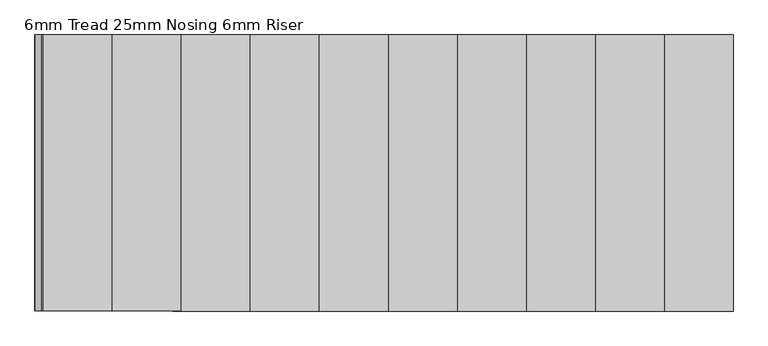
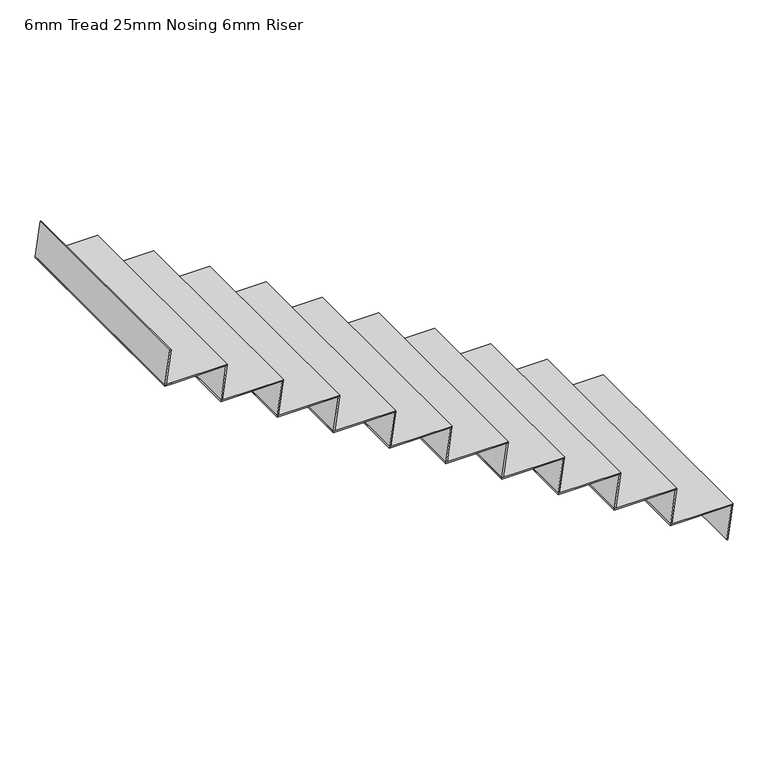
"""IFC4 building model written with IfcOpenShell, lengths in millimetres: stair flight geometry, 6mm Tread 25mm Nosing 6mm Riser."""

from ifc_helpers import new_model, si_unit, origin, place, context, project, spatial, faceted_brep, source, transform, mapped, element, save


def stair_flight_6mm_tread_25mm_nosing_6mm_riser_dd6273b0(model_context):
    return source(origin(), model_context, "Body", "Brep", [
        faceted_brep([(-13906.0599092, 11470.4345331, 8176.4705882), (-13906.9099092, 11470.4345331, 8170.4705882), (-13906.9099092, 10370.4345331, 8170.4705882), (-13906.0599092, 10370.4345331, 8176.4705882), (-13600.0, 10370.4345331, 8176.4705882), (-13600.0, 11470.4345331, 8176.4705882), (-13600.85, 11470.4345331, 8170.4705882), (-13600.85, 10370.4345331, 8170.4705882)], [[[0, 1, 2, 3]], [[3, 4, 5, 0]], [[2, 1, 6, 7]], [[4, 3, 2, 7]], [[0, 5, 6, 1]], [[5, 4, 7, 6]]]),
        faceted_brep([(-13600.85, 11470.4345331, 8170.4705882), (-13625.0, 11470.4345331, 8000.0), (-13631.0599092, 11470.4345331, 8000.0), (-13606.9099092, 11470.4345331, 8170.4705882), (-13600.85, 10370.4345331, 8170.4705882), (-13606.9099092, 10370.4345331, 8170.4705882), (-13631.0599092, 10370.4345331, 8000.0), (-13625.0, 10370.4345331, 8000.0)], [[[0, 1, 2, 3]], [[4, 5, 6, 7]], [[1, 0, 4, 7]], [[2, 1, 7, 6]], [[3, 2, 6, 5]], [[0, 3, 5, 4]]]),
        faceted_brep([(-13875.85, 11470.4345331, 8346.9411765), (-13900.0, 11470.4345331, 8176.4705882), (-13906.0599092, 11470.4345331, 8176.4705882), (-13881.9099092, 11470.4345331, 8346.9411765), (-13875.85, 10370.4345331, 8346.9411765), (-13881.9099092, 10370.4345331, 8346.9411765), (-13906.0599092, 10370.4345331, 8176.4705882), (-13900.0, 10370.4345331, 8176.4705882)], [[[0, 1, 2, 3]], [[4, 5, 6, 7]], [[1, 0, 4, 7]], [[2, 1, 7, 6]], [[3, 2, 6, 5]], [[0, 3, 5, 4]]]),
        faceted_brep([(-14181.0599092, 10370.4345331, 8352.9411765), (-13875.0, 10370.4345331, 8352.9411765), (-13875.0, 11470.4345331, 8352.9411765), (-14181.0599092, 11470.4345331, 8352.9411765), (-14181.9099092, 10370.4345331, 8346.9411765), (-14181.9099092, 11470.4345331, 8346.9411765), (-13875.85, 11470.4345331, 8346.9411765), (-13875.85, 10370.4345331, 8346.9411765)], [[[0, 1, 2, 3]], [[4, 5, 6, 7]], [[1, 0, 4, 7]], [[3, 2, 6, 5]], [[3, 5, 4, 0]], [[2, 1, 7, 6]]]),
        faceted_brep([(-14150.85, 11470.4345331, 8523.4117647), (-14175.0, 11470.4345331, 8352.9411765), (-14181.0599092, 11470.4345331, 8352.9411765), (-14156.9099092, 11470.4345331, 8523.4117647), (-14150.85, 10370.4345331, 8523.4117647), (-14156.9099092, 10370.4345331, 8523.4117647), (-14181.0599092, 10370.4345331, 8352.9411765), (-14175.0, 10370.4345331, 8352.9411765)], [[[0, 1, 2, 3]], [[4, 5, 6, 7]], [[1, 0, 4, 7]], [[2, 1, 7, 6]], [[3, 2, 6, 5]], [[0, 3, 5, 4]]]),
        faceted_brep([(-14456.0599092, 10370.4345331, 8529.4117647), (-14150.0, 10370.4345331, 8529.4117647), (-14150.0, 11470.4345331, 8529.4117647), (-14456.0599092, 11470.4345331, 8529.4117647), (-14456.9099092, 10370.4345331, 8523.4117647), (-14456.9099092, 11470.4345331, 8523.4117647), (-14150.85, 11470.4345331, 8523.4117647), (-14150.85, 10370.4345331, 8523.4117647)], [[[0, 1, 2, 3]], [[4, 5, 6, 7]], [[1, 0, 4, 7]], [[3, 2, 6, 5]], [[3, 5, 4, 0]], [[2, 1, 7, 6]]]),
        faceted_brep([(-14425.85, 11470.4345331, 8699.8823529), (-14450.0, 11470.4345331, 8529.4117647), (-14456.0599092, 11470.4345331, 8529.4117647), (-14431.9099092, 11470.4345331, 8699.8823529), (-14425.85, 10370.4345331, 8699.8823529), (-14431.9099092, 10370.4345331, 8699.8823529), (-14456.0599092, 10370.4345331, 8529.4117647), (-14450.0, 10370.4345331, 8529.4117647)], [[[0, 1, 2, 3]], [[4, 5, 6, 7]], [[1, 0, 4, 7]], [[2, 1, 7, 6]], [[3, 2, 6, 5]], [[0, 3, 5, 4]]]),
        faceted_brep([(-14731.0599092, 10370.4345331, 8705.8823529), (-14425.0, 10370.4345331, 8705.8823529), (-14425.0, 11470.4345331, 8705.8823529), (-14731.0599092, 11470.4345331, 8705.8823529), (-14731.9099092, 10370.4345331, 8699.8823529), (-14731.9099092, 11470.4345331, 8699.8823529), (-14425.85, 11470.4345331, 8699.8823529), (-14425.85, 10370.4345331, 8699.8823529)], [[[0, 1, 2, 3]], [[4, 5, 6, 7]], [[1, 0, 4, 7]], [[3, 2, 6, 5]], [[3, 5, 4, 0]], [[2, 1, 7, 6]]]),
        faceted_brep([(-14700.85, 11470.4345331, 8876.3529412), (-14725.0, 11470.4345331, 8705.8823529), (-14731.0599092, 11470.4345331, 8705.8823529), (-14706.9099092, 11470.4345331, 8876.3529412), (-14700.85, 10370.4345331, 8876.3529412), (-14706.9099092, 10370.4345331, 8876.3529412), (-14731.0599092, 10370.4345331, 8705.8823529), (-14725.0, 10370.4345331, 8705.8823529)], [[[0, 1, 2, 3]], [[4, 5, 6, 7]], [[1, 0, 4, 7]], [[2, 1, 7, 6]], [[3, 2, 6, 5]], [[0, 3, 5, 4]]]),
        faceted_brep([(-15006.0599092, 10370.4345331, 8882.3529412), (-14700.0, 10370.4345331, 8882.3529412), (-14700.0, 11470.4345331, 8882.3529412), (-15006.0599092, 11470.4345331, 8882.3529412), (-15006.9099092, 10370.4345331, 8876.3529412), (-15006.9099092, 11470.4345331, 8876.3529412), (-14700.85, 11470.4345331, 8876.3529412), (-14700.85, 10370.4345331, 8876.3529412)], [[[0, 1, 2, 3]], [[4, 5, 6, 7]], [[1, 0, 4, 7]], [[3, 2, 6, 5]], [[3, 5, 4, 0]], [[2, 1, 7, 6]]]),
        faceted_brep([(-14975.85, 11470.4345331, 9052.8235294), (-15000.0, 11470.4345331, 8882.3529412), (-15006.0599092, 11470.4345331, 8882.3529412), (-14981.9099092, 11470.4345331, 9052.8235294), (-14975.85, 10370.4345331, 9052.8235294), (-14981.9099092, 10370.4345331, 9052.8235294), (-15006.0599092, 10370.4345331, 8882.3529412), (-15000.0, 10370.4345331, 8882.3529412)], [[[0, 1, 2, 3]], [[4, 5, 6, 7]], [[1, 0, 4, 7]], [[2, 1, 7, 6]], [[3, 2, 6, 5]], [[0, 3, 5, 4]]]),
        faceted_brep([(-15281.0599092, 10370.4345331, 9058.8235294), (-14975.0, 10370.4345331, 9058.8235294), (-14975.0, 11470.4345331, 9058.8235294), (-15281.0599092, 11470.4345331, 9058.8235294), (-15281.9099092, 10370.4345331, 9052.8235294), (-15281.9099092, 11470.4345331, 9052.8235294), (-14975.85, 11470.4345331, 9052.8235294), (-14975.85, 10370.4345331, 9052.8235294)], [[[0, 1, 2, 3]], [[4, 5, 6, 7]], [[1, 0, 4, 7]], [[3, 2, 6, 5]], [[3, 5, 4, 0]], [[2, 1, 7, 6]]]),
        faceted_brep([(-15250.85, 11470.4345331, 9229.2941176), (-15275.0, 11470.4345331, 9058.8235294), (-15281.0599092, 11470.4345331, 9058.8235294), (-15256.9099092, 11470.4345331, 9229.2941176), (-15250.85, 10370.4345331, 9229.2941176), (-15256.9099092, 10370.4345331, 9229.2941176), (-15281.0599092, 10370.4345331, 9058.8235294), (-15275.0, 10370.4345331, 9058.8235294)], [[[0, 1, 2, 3]], [[4, 5, 6, 7]], [[1, 0, 4, 7]], [[2, 1, 7, 6]], [[3, 2, 6, 5]], [[0, 3, 5, 4]]]),
        faceted_brep([(-15556.0599092, 10370.4345331, 9235.2941176), (-15250.0, 10370.4345331, 9235.2941176), (-15250.0, 11470.4345331, 9235.2941176), (-15556.0599092, 11470.4345331, 9235.2941176), (-15556.9099092, 10370.4345331, 9229.2941176), (-15556.9099092, 11470.4345331, 9229.2941176), (-15250.85, 11470.4345331, 9229.2941176), (-15250.85, 10370.4345331, 9229.2941176)], [[[0, 1, 2, 3]], [[4, 5, 6, 7]], [[1, 0, 4, 7]], [[3, 2, 6, 5]], [[3, 5, 4, 0]], [[2, 1, 7, 6]]]),
        faceted_brep([(-15525.85, 11470.4345331, 9405.7647059), (-15550.0, 11470.4345331, 9235.2941176), (-15556.0599092, 11470.4345331, 9235.2941176), (-15531.9099092, 11470.4345331, 9405.7647059), (-15525.85, 10370.4345331, 9405.7647059), (-15531.9099092, 10370.4345331, 9405.7647059), (-15556.0599092, 10370.4345331, 9235.2941176), (-15550.0, 10370.4345331, 9235.2941176)], [[[0, 1, 2, 3]], [[4, 5, 6, 7]], [[1, 0, 4, 7]], [[2, 1, 7, 6]], [[3, 2, 6, 5]], [[0, 3, 5, 4]]]),
        faceted_brep([(-15831.0599092, 10370.4345331, 9411.7647059), (-15525.0, 10370.4345331, 9411.7647059), (-15525.0, 11470.4345331, 9411.7647059), (-15831.0599092, 11470.4345331, 9411.7647059), (-15831.9099092, 10370.4345331, 9405.7647059), (-15831.9099092, 11470.4345331, 9405.7647059), (-15525.85, 11470.4345331, 9405.7647059), (-15525.85, 10370.4345331, 9405.7647059)], [[[0, 1, 2, 3]], [[4, 5, 6, 7]], [[1, 0, 4, 7]], [[3, 2, 6, 5]], [[3, 5, 4, 0]], [[2, 1, 7, 6]]]),
        faceted_brep([(-15800.85, 11470.4345331, 9582.2352941), (-15825.0, 11470.4345331, 9411.7647059), (-15831.0599092, 11470.4345331, 9411.7647059), (-15806.9099092, 11470.4345331, 9582.2352941), (-15800.85, 10370.4345331, 9582.2352941), (-15806.9099092, 10370.4345331, 9582.2352941), (-15831.0599092, 10370.4345331, 9411.7647059), (-15825.0, 10370.4345331, 9411.7647059)], [[[0, 1, 2, 3]], [[4, 5, 6, 7]], [[1, 0, 4, 7]], [[2, 1, 7, 6]], [[3, 2, 6, 5]], [[0, 3, 5, 4]]]),
        faceted_brep([(-16106.0599092, 10370.4345331, 9588.2352941), (-15800.0, 10370.4345331, 9588.2352941), (-15800.0, 11470.4345331, 9588.2352941), (-16106.0599092, 11470.4345331, 9588.2352941), (-16106.9099092, 10370.4345331, 9582.2352941), (-16106.9099092, 11470.4345331, 9582.2352941), (-15800.85, 11470.4345331, 9582.2352941), (-15800.85, 10370.4345331, 9582.2352941)], [[[0, 1, 2, 3]], [[4, 5, 6, 7]], [[1, 0, 4, 7]], [[3, 2, 6, 5]], [[3, 5, 4, 0]], [[2, 1, 7, 6]]]),
        faceted_brep([(-16075.85, 11470.4345331, 9758.7058824), (-16100.0, 11470.4345331, 9588.2352941), (-16106.0599092, 11470.4345331, 9588.2352941), (-16081.9099092, 11470.4345331, 9758.7058824), (-16075.85, 10370.4345331, 9758.7058824), (-16081.9099092, 10370.4345331, 9758.7058824), (-16106.0599092, 10370.4345331, 9588.2352941), (-16100.0, 10370.4345331, 9588.2352941)], [[[0, 1, 2, 3]], [[4, 5, 6, 7]], [[1, 0, 4, 7]], [[2, 1, 7, 6]], [[3, 2, 6, 5]], [[0, 3, 5, 4]]]),
        faceted_brep([(-16350.85, 11470.4345331, 9935.1764706), (-16375.0, 11470.4345331, 9764.7058824), (-16381.0599092, 11470.4345331, 9764.7058824), (-16356.9099092, 11470.4345331, 9935.1764706), (-16350.85, 10370.4345331, 9935.1764706), (-16356.9099092, 10370.4345331, 9935.1764706), (-16381.0599092, 10370.4345331, 9764.7058824), (-16375.0, 10370.4345331, 9764.7058824)], [[[0, 1, 2, 3]], [[4, 5, 6, 7]], [[1, 0, 4, 7]], [[2, 1, 7, 6]], [[3, 2, 6, 5]], [[0, 3, 5, 4]]]),
        faceted_brep([(-16381.0599092, 10370.4345331, 9764.7058824), (-16350.0, 10370.4345331, 9764.7058824), (-16075.0, 10370.4345331, 9764.7058824), (-16075.0, 11470.4345331, 9764.7058824), (-16381.0599092, 11470.4345331, 9764.7058824), (-16381.9099092, 10370.4345331, 9758.7058824), (-16381.9099092, 11470.4345331, 9758.7058824), (-16075.85, 11470.4345331, 9758.7058824), (-16075.85, 10370.4345331, 9758.7058824), (-16350.0, 10370.4345331, 9758.7058824)], [[[0, 1, 2, 3, 4]], [[5, 6, 7, 8, 9]], [[1, 0, 5, 9]], [[2, 1, 9, 8]], [[4, 3, 7, 6]], [[4, 6, 5, 0]], [[3, 2, 8, 7]]]),
    ])


if __name__ == "__main__":
    model = new_model("IFC4")
    model_context = context("Model", 3, world=origin())
    ifc_project = project(units=[si_unit("LENGTHUNIT", "METRE", prefix="MILLI")], contexts=[model_context])
    site = spatial("IfcSite", under=ifc_project)
    building = spatial("IfcBuilding", under=site)
    placement = place(None, origin())
    stair_flight_6mm_tread_25mm_nosing_6mm_riser_shape = stair_flight_6mm_tread_25mm_nosing_6mm_riser_dd6273b0(model_context)
    element("IfcStairFlight", 1, ObjectType="6mm Tread 25mm Nosing 6mm Riser", at=placement, inside=building, context=model_context, shape_type="MappedRepresentation", body=[
        mapped(stair_flight_6mm_tread_25mm_nosing_6mm_riser_shape, transform((0.0, 0.0, 0.0), x_axis=(1.0, 0.0, 0.0), y_axis=(0.0, 1.0, 0.0), z_axis=(0.0, 0.0, 1.0))),
    ])
    save(model, "model.ifc")

# Revit data of these elements
# Element 1 (IfcStairFlight, "6mm Tread 25mm Nosing 6mm Riser")
#   Materials on its faces: "Steel, Paint Finish, Dark Gray"
# Materials
#   "Steel, Paint Finish, Dark Gray": class "Metal", colour RGB 89 89 89, transparency 0, Description = "Steel, paint finish, dark gray, glossy", Cost = 0
